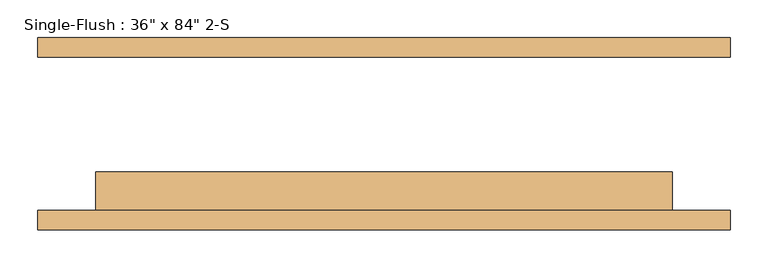
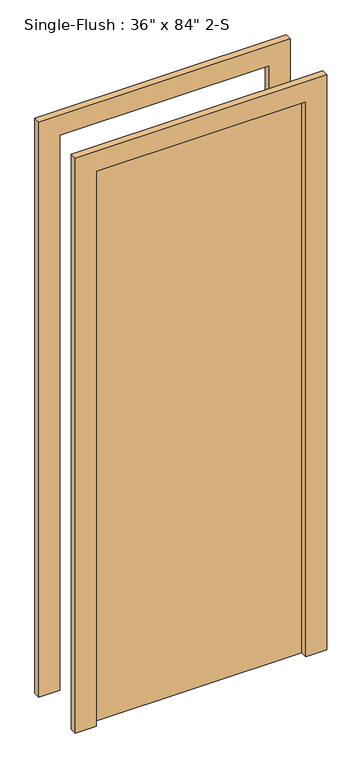
"""IFC4 building model written with IfcOpenShell, lengths in millimetres: door geometry."""

from ifc_helpers import new_model, si_unit, frame, origin, origin_with_axes, place, context, project, spatial, polyline, outline, extrude, source, transform, mapped, element, save


def door_4314e8ec(model_context):
    return source(origin(), model_context, "Body", "SweptSolid", [
        extrude(outline(polyline([(2209.8, -457.2), (0.0, -457.2), (0.0, -381.0), (2133.6, -381.0), (2133.6, 381.0), (0.0, 381.0), (0.0, 457.2), (2209.8, 457.2), (2209.8, -457.2)])), frame((0.0, -127.0, 0.0), z_axis=(0.0, 1.0, 0.0), x_axis=(0.0, 0.0, 1.0)), (0.0, 0.0, 1.0), 25.4),
        extrude(outline(polyline([(2209.8, 457.2), (2209.8, -457.2), (0.0, -457.2), (0.0, -381.0), (2133.6, -381.0), (2133.6, 381.0), (0.0, 381.0), (0.0, 457.2), (2209.8, 457.2)])), frame((0.0, 101.6, 0.0), z_axis=(0.0, 1.0, 0.0), x_axis=(0.0, 0.0, 1.0)), (0.0, 0.0, 1.0), 25.4),
        extrude(outline(polyline([(381.0, -50.8), (381.0, -101.6), (-381.0, -101.6), (-381.0, -50.8), (381.0, -50.8)])), origin_with_axes(), (0.0, 0.0, 1.0), 2133.6),
    ])


if __name__ == "__main__":
    model = new_model("IFC4")
    model_context = context("Model", 3, world=origin())
    ifc_project = project(units=[si_unit("LENGTHUNIT", "METRE", prefix="MILLI")], contexts=[model_context])
    site = spatial("IfcSite", under=ifc_project)
    building = spatial("IfcBuilding", under=site)
    placement = place(None, origin())
    door_shape = door_4314e8ec(model_context)
    element("IfcDoor", 1, ObjectType="Single-Flush : 36\" x 84\" 2-S", at=placement, inside=building, context=model_context, shape_type="MappedRepresentation", body=[
        mapped(door_shape, transform((0.0, 0.0, 0.0), x_axis=(1.0, 0.0, 0.0), y_axis=(0.0, 1.0, 0.0), z_axis=(0.0, 0.0, 1.0))),
    ])
    save(model, "model.ifc")

# Revit data of these elements
# Type "Single-Flush : 36\" x 84\" 2-S"
#   Type Mark = "57"
#   Assembly Code = "C1020"
#   Thickness = 0' - 2"
#   Height = 7' - 0"
#   Trim Projection Ext = 0' - 1"
#   Trim Projection Int = 0' - 1"
#   Trim Width = 0' - 3"
#   Width = 2' - 6"
#   Door Material = Door - Panel
#   Frame Material = Door - Frame
#   Wall Closure = (empty or 0)
# Element 1 (IfcDoor, "Single-Flush : 36\" x 84\" 2-S")
#   Materials on its faces: "Door - Frame", "Door - Panel"
# Materials
#   "Door - Panel": class "Wood", colour RGB 227 170 128, transparency 0, Cost = 0
#   "Door - Frame": class "Miscellaneous", colour RGB 153 76 43, transparency 0, Cost = 0
